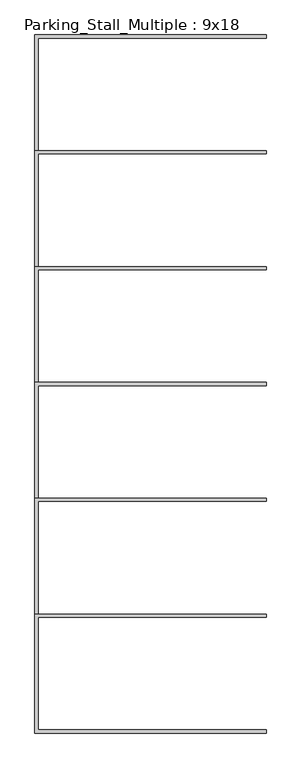
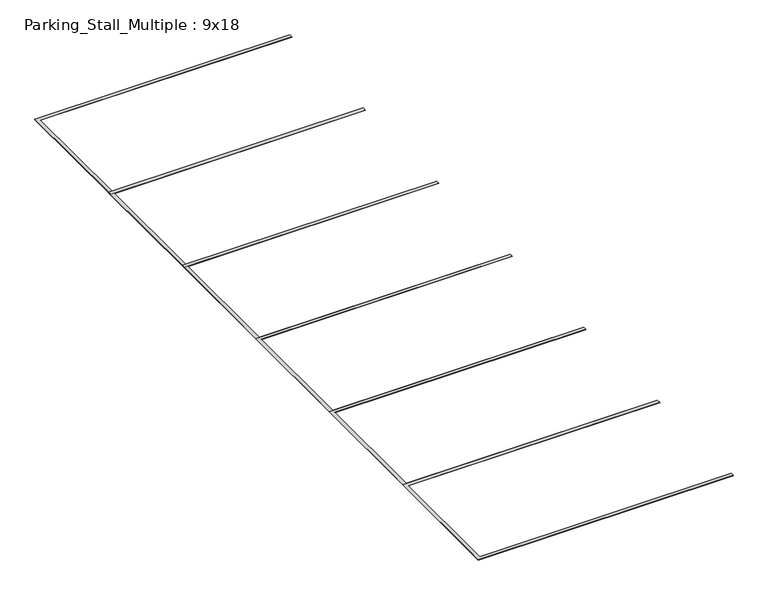
"""IFC4 building model written with IfcOpenShell, lengths in millimetres: proxy geometry, Parking_Stall_Multiple : 9x18."""

from ifc_helpers import new_model, si_unit, origin, origin_with_axes, place, context, project, spatial, polyline, outline, extrude, source, transform, mapped, element, save


def parking_stall_multiple_9x18_c8fa3216(model_context):
    return source(origin(), model_context, "Body", "SweptSolid", [
        extrude(outline(polyline([(5486.4, -13716.0), (5486.4, -13792.2), (76.2, -13792.2), (76.2, -16459.2), (5486.4, -16459.2), (5486.4, -16535.4), (0.0, -16535.4), (0.0, -13716.0), (5486.4, -13716.0)])), origin_with_axes(), (0.0, 0.0, 1.0), 6.35),
        extrude(outline(polyline([(5486.4, -10972.8), (5486.4, -11049.0), (76.2, -11049.0), (76.2, -13716.0), (5486.4, -13716.0), (5486.4, -13792.2), (0.0, -13792.2), (0.0, -10972.8), (5486.4, -10972.8)])), origin_with_axes(), (0.0, 0.0, 1.0), 6.35),
        extrude(outline(polyline([(5486.4, -8229.6), (5486.4, -8305.8), (76.2, -8305.8), (76.2, -10972.8), (5486.4, -10972.8), (5486.4, -11049.0), (0.0, -11049.0), (0.0, -8229.6), (5486.4, -8229.6)])), origin_with_axes(), (0.0, 0.0, 1.0), 6.35),
        extrude(outline(polyline([(5486.4, -5486.4), (5486.4, -5562.6), (76.2, -5562.6), (76.2, -8229.6), (5486.4, -8229.6), (5486.4, -8305.8), (0.0, -8305.8), (0.0, -5486.4), (5486.4, -5486.4)])), origin_with_axes(), (0.0, 0.0, 1.0), 6.35),
        extrude(outline(polyline([(5486.4, -2743.2), (5486.4, -2819.4), (76.2, -2819.4), (76.2, -5486.4), (5486.4, -5486.4), (5486.4, -5562.6), (0.0, -5562.6), (0.0, -2743.2), (5486.4, -2743.2)])), origin_with_axes(), (0.0, 0.0, 1.0), 6.35),
        extrude(outline(polyline([(5486.4, 0.0), (5486.4, -76.2), (76.2, -76.2), (76.2, -2743.2), (5486.4, -2743.2), (5486.4, -2819.4), (0.0, -2819.4), (0.0, 0.0), (5486.4, 0.0)])), origin_with_axes(), (0.0, 0.0, 1.0), 6.35),
    ])


if __name__ == "__main__":
    model = new_model("IFC4")
    model_context = context("Model", 3, world=origin())
    ifc_project = project(units=[si_unit("LENGTHUNIT", "METRE", prefix="MILLI")], contexts=[model_context])
    site = spatial("IfcSite", under=ifc_project)
    building = spatial("IfcBuilding", under=site)
    placement = place(None, origin())
    parking_stall_multiple_9x18_shape = parking_stall_multiple_9x18_c8fa3216(model_context)
    element("IfcBuildingElementProxy", 1, Name="Parking_Stall_Multiple : 9x18", ObjectType="Parking_Stall_Multiple : 9x18", at=placement, inside=building, context=model_context, shape_type="MappedRepresentation", body=[
        mapped(parking_stall_multiple_9x18_shape, transform((0.0, 0.0, 0.0), x_axis=(1.0, 0.0, 0.0), y_axis=(0.0, 1.0, 0.0), z_axis=(0.0, 0.0, 1.0))),
    ])
    save(model, "model.ifc")

# Revit data of these elements
# Type "Parking_Stall_Multiple : 9x18"
#   Type Mark = "PK-1"
#   Parking_Width_M = 9' - 0"
#   Parking_Run_Length [instance default] = 65' - 0"
#   Parking_Line_Width = 0' - 3"
#   Parking_Length_M = 18' - 0"
#   Single_Parking_Visibility [instance default] = no
#   Parking_ADA_Symbol = no
#   ParkingUnitsArray [instance default] = 7
#   ParkingUnits [instance default] = 7
#   Multiple_Parking_Visibility [instance default] = yes
#   Parking_Line_Material = none
# Element 1 (IfcBuildingElementProxy, "Parking_Stall_Multiple : 9x18")
#   Parking_Run_Length = 55' - 2.5365"
#   ParkingUnitsArray = 6
#   ParkingUnits = 6
